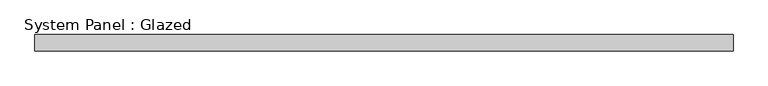
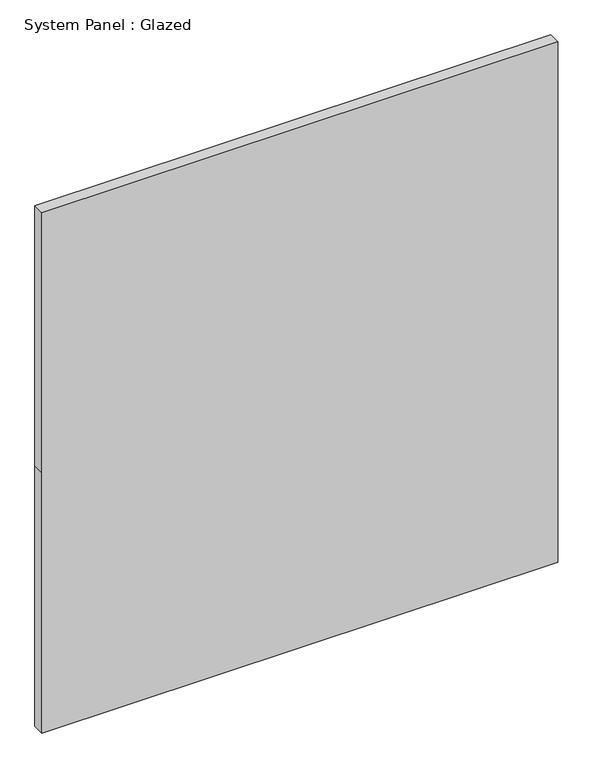
"""IFC4 building model written with IfcOpenShell, lengths in millimetres: plate geometry, System Panel : Glazed."""

import ifcopenshell
import ifcopenshell.guid

model = None  # the IFC model being written
_history = None  # IfcOwnerHistory: only IFC2X3 demands one
_inside = {}  # id of a spatial element -> (the spatial element, [elements in it])
_under = {}  # id of a project, library or spatial element -> (it, [spatial elements below it])
_declared = {}  # id of a project -> (the project, [libraries it declares])
_typed = {}  # id of a type object -> (the type object, [elements of that type])
_made_of = {}  # id of a material, layer set ... -> (it, [elements and type objects made of it])


def new_model(schema):
    """Start an empty IFC model of exactly this schema.

    Asked for "IFC4X3", IfcOpenShell would pick the latest addendum, in which some entities
    have other attributes; the version numbers below select the first issue.
    IFC2X3 requires an IfcOwnerHistory on every rooted entity: one is made here for all.
    """
    global model, _history
    if schema == "IFC4X3":
        model = ifcopenshell.file(schema_version=(4, 3, 0, 0))
    else:
        model = ifcopenshell.file(schema=schema)
    _inside.clear()
    _under.clear()
    _declared.clear()
    _typed.clear()
    _made_of.clear()
    _history = None
    if model.schema == "IFC2X3":
        org = make("IfcOrganization", Name="unknown")
        user = make(
            "IfcPersonAndOrganization",
            ThePerson=make("IfcPerson", FamilyName="unknown"),
            TheOrganization=org,
        )
        app = make(
            "IfcApplication",
            ApplicationDeveloper=org,
            Version="unknown",
            ApplicationFullName="unknown",
            ApplicationIdentifier="unknown",
        )
        _history = make(
            "IfcOwnerHistory",
            OwningUser=user,
            OwningApplication=app,
            ChangeAction="ADDED",
            CreationDate=0,
        )
    return model


def make(cls, **values):
    """One entity of the class cls with the attributes given. An attribute that is None is left unset."""
    return model.create_entity(
        cls, **{name: value for name, value in values.items() if value is not None}
    )


def rooted(cls, **values):
    """An entity with a GlobalId (a new one), such as an element, a storey or a relation."""
    return make(cls, GlobalId=ifcopenshell.guid.new(), OwnerHistory=_history, **values)


def si_unit(unit_type, name, prefix=None):
    """IfcSIUnit, for example si_unit("LENGTHUNIT", "METRE", prefix="MILLI")."""
    return make("IfcSIUnit", UnitType=unit_type, Prefix=prefix, Name=name)


def assignment(units):
    """IfcUnitAssignment: the units of a project."""
    return None if units is None else make("IfcUnitAssignment", Units=units)


def point(xyz):
    """IfcCartesianPoint."""
    return None if xyz is None else make("IfcCartesianPoint", Coordinates=xyz)


def direction(xyz):
    """IfcDirection."""
    return None if xyz is None else make("IfcDirection", DirectionRatios=xyz)


def frame(location, z_axis=None, x_axis=None):
    """IfcAxis2Placement3D, a coordinate frame: its origin and axes. An axis left out is left unset."""
    return make(
        "IfcAxis2Placement3D",
        Location=point(location),
        Axis=direction(z_axis),
        RefDirection=direction(x_axis),
    )


def origin():
    """The frame at (0, 0, 0) with its axes left unset."""
    return frame((0.0, 0.0, 0.0))


def place(relative_to, where):
    """IfcLocalPlacement: puts the frame where relative to a parent placement (None: the world)."""
    return make(
        "IfcLocalPlacement", PlacementRelTo=relative_to, RelativePlacement=where
    )


def context(
    kind, dimensions, precision=None, world=None, true_north=None, identifier=None
):
    """IfcGeometricRepresentationContext, for example the 3D "Model" context."""
    return make(
        "IfcGeometricRepresentationContext",
        ContextIdentifier=identifier,
        ContextType=kind,
        CoordinateSpaceDimension=dimensions,
        Precision=precision,
        WorldCoordinateSystem=world,
        TrueNorth=true_north,
    )


def project(units=None, contexts=None):
    """IfcProject with its units and contexts."""
    return rooted(
        "IfcProject",
        Name="project",
        RepresentationContexts=contexts,
        UnitsInContext=assignment(units),
    )


def spatial(cls, under=None, at=None, **own):
    """A site, building, storey or space (cls), placed at a placement, below another one or the project."""
    s = rooted(cls, ObjectPlacement=at, **own)
    if under is not None:
        _under.setdefault(under.id(), (under, []))[1].append(s)
    return s


def polyline(points):
    """IfcPolyline through the points."""
    return make("IfcPolyline", Points=[point(p) for p in points])


def outline(outer, holes=None, kind="AREA"):
    """IfcArbitraryClosedProfileDef: a profile drawn as a closed curve; with holes, ...WithVoids."""
    if holes is None:
        return make("IfcArbitraryClosedProfileDef", ProfileType=kind, OuterCurve=outer)
    return make(
        "IfcArbitraryProfileDefWithVoids",
        ProfileType=kind,
        OuterCurve=outer,
        InnerCurves=holes,
    )


def extrude(swept, where, along, depth):
    """IfcExtrudedAreaSolid: the profile swept, set in the frame where, extruded along a direction by depth."""
    return make(
        "IfcExtrudedAreaSolid",
        SweptArea=swept,
        Position=where,
        ExtrudedDirection=direction(along),
        Depth=depth,
    )


def shape(context_of_items, identifier, shape_type, items):
    """IfcShapeRepresentation: the items that make up one representation, for example the "Body"."""
    return make(
        "IfcShapeRepresentation",
        ContextOfItems=context_of_items,
        RepresentationIdentifier=identifier,
        RepresentationType=shape_type,
        Items=items,
    )


def source(mapping_origin, context_of_items, identifier, shape_type, items):
    """IfcRepresentationMap: a shape defined once, which mapped items show again and again."""
    return make(
        "IfcRepresentationMap",
        MappingOrigin=mapping_origin,
        MappedRepresentation=shape(context_of_items, identifier, shape_type, items),
    )


def transform(
    local_origin,
    x_axis=None,
    y_axis=None,
    z_axis=None,
    scale=None,
    scale2=None,
    scale3=None,
    uniform=True,
):
    """IfcCartesianTransformationOperator3D, or its non-uniform kind. x_axis, y_axis, z_axis: its Axis1, 2, 3."""
    if uniform:
        return make(
            "IfcCartesianTransformationOperator3D",
            Axis1=direction(x_axis),
            Axis2=direction(y_axis),
            LocalOrigin=point(local_origin),
            Scale=scale,
            Axis3=direction(z_axis),
        )
    return make(
        "IfcCartesianTransformationOperator3DnonUniform",
        Axis1=direction(x_axis),
        Axis2=direction(y_axis),
        LocalOrigin=point(local_origin),
        Scale=scale,
        Axis3=direction(z_axis),
        Scale2=scale2,
        Scale3=scale3,
    )


def mapped(mapping_source, mapping_target):
    """IfcMappedItem: shows the shape of a source again, moved by a transform."""
    return make(
        "IfcMappedItem", MappingSource=mapping_source, MappingTarget=mapping_target
    )


def made_of(thing, what):
    """Note that an element or type object is made of a material, layer set ...; save() writes the relation."""
    if what is not None:
        _made_of.setdefault(what.id(), (what, []))[1].append(thing)
    return thing


def element(
    cls,
    number,
    at=None,
    inside=None,
    cuts=None,
    type_object=None,
    material=None,
    context=None,
    identifier="Body",
    shape_type=None,
    held_by="IfcProductDefinitionShape",
    body=None,
    shapes=None,
    **own,
):
    """One element of the class cls, such as IfcWall. Its Tag is "e" and its number.

    at: its placement. inside: the storey or other place that contains it. cuts: it is an
    opening in that element (IfcRelVoidsElement). A single representation is given by context,
    identifier, shape_type and body (its items); several are given by shapes. held_by: the class
    of the entity that holds the representations. save() writes the other relations.
    """
    e = rooted(cls, Tag="e%d" % number, ObjectPlacement=at, **own)
    if body is not None:
        shapes = [shape(context, identifier, shape_type, body)]
    if shapes is not None:
        e.Representation = make(held_by, Representations=shapes)
    if inside is not None:
        _inside.setdefault(inside.id(), (inside, []))[1].append(e)
    if cuts is not None:
        rooted(
            "IfcRelVoidsElement", RelatingBuildingElement=cuts, RelatedOpeningElement=e
        )
    if type_object is not None:
        _typed.setdefault(type_object.id(), (type_object, []))[1].append(e)
    return made_of(e, material)


def aggregate(whole, parts):
    """IfcRelAggregates: a whole, such as a stair, and the parts it consists of."""
    return rooted("IfcRelAggregates", RelatingObject=whole, RelatedObjects=parts)


def save(model, path):
    """Write the relations noted so far, then the file.

    IfcRelAggregates (storeys below a building ...), IfcRelContainedInSpatialStructure (elements
    in a storey), IfcRelDefinesByType, IfcRelAssociatesMaterial and IfcRelDeclares: one each for
    every whole, place, type object, material and project.
    """
    for whole, parts in _under.values():
        aggregate(whole, parts)
    for where, things in _inside.values():
        rooted(
            "IfcRelContainedInSpatialStructure",
            RelatedElements=things,
            RelatingStructure=where,
        )
    for kind, things in _typed.values():
        rooted("IfcRelDefinesByType", RelatedObjects=things, RelatingType=kind)
    for what, things in _made_of.values():
        rooted("IfcRelAssociatesMaterial", RelatedObjects=things, RelatingMaterial=what)
    for by, libraries in _declared.values():
        rooted("IfcRelDeclares", RelatingContext=by, RelatedDefinitions=libraries)
    model.write(path)


def system_panel_glazed_9400200b(model_context):
    return source(origin(), model_context, "Body", "SweptSolid", [
        extrude(outline(polyline([(0.0, -541.655), (0.0, 541.655), (577.85, 541.655), (1155.7, 541.655), (1155.7, -541.655), (577.85, -541.655), (0.0, -541.655)])), frame((0.0, -44.45, 0.0), z_axis=(0.0, 1.0, 0.0), x_axis=(0.0, 0.0, 1.0)), (0.0, 0.0, 1.0), 25.4),
    ])


if __name__ == "__main__":
    model = new_model("IFC4")
    model_context = context("Model", 3, world=origin())
    ifc_project = project(units=[si_unit("LENGTHUNIT", "METRE", prefix="MILLI")], contexts=[model_context])
    site = spatial("IfcSite", under=ifc_project)
    building = spatial("IfcBuilding", under=site)
    placement = place(None, origin())
    system_panel_glazed_shape = system_panel_glazed_9400200b(model_context)
    element("IfcPlate", 1, ObjectType="System Panel : Glazed", at=placement, inside=building, context=model_context, shape_type="MappedRepresentation", body=[
        mapped(system_panel_glazed_shape, transform((0.0, 0.0, 0.0), x_axis=(1.0, 0.0, 0.0), y_axis=(0.0, 1.0, 0.0), z_axis=(0.0, 0.0, 1.0))),
    ])
    save(model, "model.ifc")

# Revit data of these elements
# Element 1 (IfcPlate, "System Panel : Glazed")
#   Materials on its faces: "Glass"
# Materials
#   "Glass": class "Unassigned", colour RGB 0 0 255, transparency 0.75
